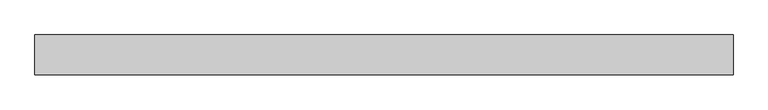
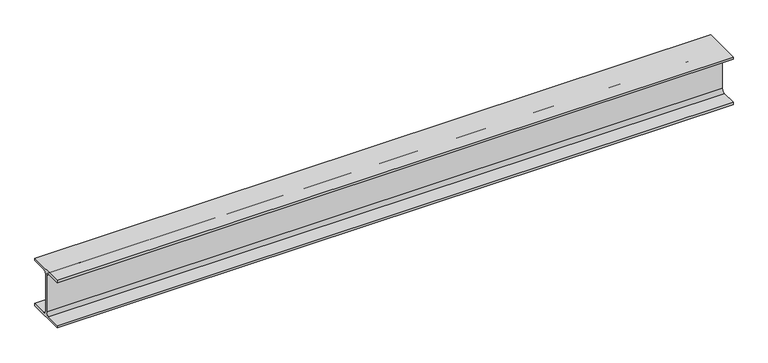
"""IFC4 building model written with IfcOpenShell, lengths in millimetres: beam geometry, 0912_Steel Framing_H-KSD3502 : H_SB_ASB_H-194x150x6x9."""

import ifcopenshell
import ifcopenshell.guid

model = None  # the IFC model being written
_history = None  # IfcOwnerHistory: only IFC2X3 demands one
_inside = {}  # id of a spatial element -> (the spatial element, [elements in it])
_under = {}  # id of a project, library or spatial element -> (it, [spatial elements below it])
_declared = {}  # id of a project -> (the project, [libraries it declares])
_typed = {}  # id of a type object -> (the type object, [elements of that type])
_made_of = {}  # id of a material, layer set ... -> (it, [elements and type objects made of it])


def new_model(schema):
    """Start an empty IFC model of exactly this schema.

    Asked for "IFC4X3", IfcOpenShell would pick the latest addendum, in which some entities
    have other attributes; the version numbers below select the first issue.
    IFC2X3 requires an IfcOwnerHistory on every rooted entity: one is made here for all.
    """
    global model, _history
    if schema == "IFC4X3":
        model = ifcopenshell.file(schema_version=(4, 3, 0, 0))
    else:
        model = ifcopenshell.file(schema=schema)
    _inside.clear()
    _under.clear()
    _declared.clear()
    _typed.clear()
    _made_of.clear()
    _history = None
    if model.schema == "IFC2X3":
        org = make("IfcOrganization", Name="unknown")
        user = make(
            "IfcPersonAndOrganization",
            ThePerson=make("IfcPerson", FamilyName="unknown"),
            TheOrganization=org,
        )
        app = make(
            "IfcApplication",
            ApplicationDeveloper=org,
            Version="unknown",
            ApplicationFullName="unknown",
            ApplicationIdentifier="unknown",
        )
        _history = make(
            "IfcOwnerHistory",
            OwningUser=user,
            OwningApplication=app,
            ChangeAction="ADDED",
            CreationDate=0,
        )
    return model


def make(cls, **values):
    """One entity of the class cls with the attributes given. An attribute that is None is left unset."""
    return model.create_entity(
        cls, **{name: value for name, value in values.items() if value is not None}
    )


def rooted(cls, **values):
    """An entity with a GlobalId (a new one), such as an element, a storey or a relation."""
    return make(cls, GlobalId=ifcopenshell.guid.new(), OwnerHistory=_history, **values)


def si_unit(unit_type, name, prefix=None):
    """IfcSIUnit, for example si_unit("LENGTHUNIT", "METRE", prefix="MILLI")."""
    return make("IfcSIUnit", UnitType=unit_type, Prefix=prefix, Name=name)


def assignment(units):
    """IfcUnitAssignment: the units of a project."""
    return None if units is None else make("IfcUnitAssignment", Units=units)


def point(xyz):
    """IfcCartesianPoint."""
    return None if xyz is None else make("IfcCartesianPoint", Coordinates=xyz)


def direction(xyz):
    """IfcDirection."""
    return None if xyz is None else make("IfcDirection", DirectionRatios=xyz)


def frame(location, z_axis=None, x_axis=None):
    """IfcAxis2Placement3D, a coordinate frame: its origin and axes. An axis left out is left unset."""
    return make(
        "IfcAxis2Placement3D",
        Location=point(location),
        Axis=direction(z_axis),
        RefDirection=direction(x_axis),
    )


def frame_2d(location, x_axis=None):
    """IfcAxis2Placement2D, a coordinate frame in the plane: its origin and x axis."""
    return make(
        "IfcAxis2Placement2D", Location=point(location), RefDirection=direction(x_axis)
    )


def origin():
    """The frame at (0, 0, 0) with its axes left unset."""
    return frame((0.0, 0.0, 0.0))


def place(relative_to, where):
    """IfcLocalPlacement: puts the frame where relative to a parent placement (None: the world)."""
    return make(
        "IfcLocalPlacement", PlacementRelTo=relative_to, RelativePlacement=where
    )


def context(
    kind, dimensions, precision=None, world=None, true_north=None, identifier=None
):
    """IfcGeometricRepresentationContext, for example the 3D "Model" context."""
    return make(
        "IfcGeometricRepresentationContext",
        ContextIdentifier=identifier,
        ContextType=kind,
        CoordinateSpaceDimension=dimensions,
        Precision=precision,
        WorldCoordinateSystem=world,
        TrueNorth=true_north,
    )


def project(units=None, contexts=None):
    """IfcProject with its units and contexts."""
    return rooted(
        "IfcProject",
        Name="project",
        RepresentationContexts=contexts,
        UnitsInContext=assignment(units),
    )


def spatial(cls, under=None, at=None, **own):
    """A site, building, storey or space (cls), placed at a placement, below another one or the project."""
    s = rooted(cls, ObjectPlacement=at, **own)
    if under is not None:
        _under.setdefault(under.id(), (under, []))[1].append(s)
    return s


def polyline(points):
    """IfcPolyline through the points."""
    return make("IfcPolyline", Points=[point(p) for p in points])


def circle_curve(where, radius):
    """IfcCircle in the frame where."""
    return make("IfcCircle", Position=where, Radius=radius)


def trimmed(basis, trim1, trim2, sense, master):
    """IfcTrimmedCurve: the piece of a basis curve between two trims."""
    return make(
        "IfcTrimmedCurve",
        BasisCurve=basis,
        Trim1=trim1,
        Trim2=trim2,
        SenseAgreement=sense,
        MasterRepresentation=master,
    )


def segment(curve, same_sense, transition):
    """IfcCompositeCurveSegment."""
    return make(
        "IfcCompositeCurveSegment",
        Transition=transition,
        SameSense=same_sense,
        ParentCurve=curve,
    )


def composite_curve(segments, self_intersect=None):
    """IfcCompositeCurve: segments joined end to end."""
    return make("IfcCompositeCurve", Segments=segments, SelfIntersect=self_intersect)


def outline(outer, holes=None, kind="AREA"):
    """IfcArbitraryClosedProfileDef: a profile drawn as a closed curve; with holes, ...WithVoids."""
    if holes is None:
        return make("IfcArbitraryClosedProfileDef", ProfileType=kind, OuterCurve=outer)
    return make(
        "IfcArbitraryProfileDefWithVoids",
        ProfileType=kind,
        OuterCurve=outer,
        InnerCurves=holes,
    )


def extrude(swept, where, along, depth):
    """IfcExtrudedAreaSolid: the profile swept, set in the frame where, extruded along a direction by depth."""
    return make(
        "IfcExtrudedAreaSolid",
        SweptArea=swept,
        Position=where,
        ExtrudedDirection=direction(along),
        Depth=depth,
    )


def shape(context_of_items, identifier, shape_type, items):
    """IfcShapeRepresentation: the items that make up one representation, for example the "Body"."""
    return make(
        "IfcShapeRepresentation",
        ContextOfItems=context_of_items,
        RepresentationIdentifier=identifier,
        RepresentationType=shape_type,
        Items=items,
    )


def source(mapping_origin, context_of_items, identifier, shape_type, items):
    """IfcRepresentationMap: a shape defined once, which mapped items show again and again."""
    return make(
        "IfcRepresentationMap",
        MappingOrigin=mapping_origin,
        MappedRepresentation=shape(context_of_items, identifier, shape_type, items),
    )


def transform(
    local_origin,
    x_axis=None,
    y_axis=None,
    z_axis=None,
    scale=None,
    scale2=None,
    scale3=None,
    uniform=True,
):
    """IfcCartesianTransformationOperator3D, or its non-uniform kind. x_axis, y_axis, z_axis: its Axis1, 2, 3."""
    if uniform:
        return make(
            "IfcCartesianTransformationOperator3D",
            Axis1=direction(x_axis),
            Axis2=direction(y_axis),
            LocalOrigin=point(local_origin),
            Scale=scale,
            Axis3=direction(z_axis),
        )
    return make(
        "IfcCartesianTransformationOperator3DnonUniform",
        Axis1=direction(x_axis),
        Axis2=direction(y_axis),
        LocalOrigin=point(local_origin),
        Scale=scale,
        Axis3=direction(z_axis),
        Scale2=scale2,
        Scale3=scale3,
    )


def mapped(mapping_source, mapping_target):
    """IfcMappedItem: shows the shape of a source again, moved by a transform."""
    return make(
        "IfcMappedItem", MappingSource=mapping_source, MappingTarget=mapping_target
    )


def made_of(thing, what):
    """Note that an element or type object is made of a material, layer set ...; save() writes the relation."""
    if what is not None:
        _made_of.setdefault(what.id(), (what, []))[1].append(thing)
    return thing


def element(
    cls,
    number,
    at=None,
    inside=None,
    cuts=None,
    type_object=None,
    material=None,
    context=None,
    identifier="Body",
    shape_type=None,
    held_by="IfcProductDefinitionShape",
    body=None,
    shapes=None,
    **own,
):
    """One element of the class cls, such as IfcWall. Its Tag is "e" and its number.

    at: its placement. inside: the storey or other place that contains it. cuts: it is an
    opening in that element (IfcRelVoidsElement). A single representation is given by context,
    identifier, shape_type and body (its items); several are given by shapes. held_by: the class
    of the entity that holds the representations. save() writes the other relations.
    """
    e = rooted(cls, Tag="e%d" % number, ObjectPlacement=at, **own)
    if body is not None:
        shapes = [shape(context, identifier, shape_type, body)]
    if shapes is not None:
        e.Representation = make(held_by, Representations=shapes)
    if inside is not None:
        _inside.setdefault(inside.id(), (inside, []))[1].append(e)
    if cuts is not None:
        rooted(
            "IfcRelVoidsElement", RelatingBuildingElement=cuts, RelatedOpeningElement=e
        )
    if type_object is not None:
        _typed.setdefault(type_object.id(), (type_object, []))[1].append(e)
    return made_of(e, material)


def aggregate(whole, parts):
    """IfcRelAggregates: a whole, such as a stair, and the parts it consists of."""
    return rooted("IfcRelAggregates", RelatingObject=whole, RelatedObjects=parts)


def save(model, path):
    """Write the relations noted so far, then the file.

    IfcRelAggregates (storeys below a building ...), IfcRelContainedInSpatialStructure (elements
    in a storey), IfcRelDefinesByType, IfcRelAssociatesMaterial and IfcRelDeclares: one each for
    every whole, place, type object, material and project.
    """
    for whole, parts in _under.values():
        aggregate(whole, parts)
    for where, things in _inside.values():
        rooted(
            "IfcRelContainedInSpatialStructure",
            RelatedElements=things,
            RelatingStructure=where,
        )
    for kind, things in _typed.values():
        rooted("IfcRelDefinesByType", RelatedObjects=things, RelatingType=kind)
    for what, things in _made_of.values():
        rooted("IfcRelAssociatesMaterial", RelatedObjects=things, RelatingMaterial=what)
    for by, libraries in _declared.values():
        rooted("IfcRelDeclares", RelatingContext=by, RelatedDefinitions=libraries)
    model.write(path)


def beam_8b6bb364(model_context):
    return source(origin(), model_context, "Body", "SweptSolid", [
        extrude(outline(composite_curve([segment(polyline([(75.0, -88.0), (75.0, -97.0), (-75.0, -97.0), (-75.0, -88.0), (-16.0, -88.0)]), True, "CONTINUOUS"), segment(trimmed(circle_curve(frame_2d((-16.0, -75.0)), 13.0), [point((-16.0, -88.0))], [point((-3.0, -75.0))], True, "CARTESIAN"), True, "CONTINUOUS"), segment(polyline([(-3.0, -75.0), (-3.0, 75.0)]), True, "CONTINUOUS"), segment(trimmed(circle_curve(frame_2d((-16.0, 75.0)), 13.0), [point((-3.0, 75.0))], [point((-16.0, 88.0))], True, "CARTESIAN"), True, "CONTINUOUS"), segment(polyline([(-16.0, 88.0), (-75.0, 88.0), (-75.0, 97.0), (75.0, 97.0), (75.0, 88.0), (16.0, 88.0)]), True, "CONTINUOUS"), segment(trimmed(circle_curve(frame_2d((16.0, 75.0)), 13.0), [point((16.0, 88.0))], [point((3.0, 75.0))], True, "CARTESIAN"), True, "CONTINUOUS"), segment(polyline([(3.0, 75.0), (3.0, -75.0)]), True, "CONTINUOUS"), segment(trimmed(circle_curve(frame_2d((16.0, -75.0)), 13.0), [point((3.0, -75.0))], [point((16.0, -88.0))], True, "CARTESIAN"), True, "CONTINUOUS"), segment(polyline([(16.0, -88.0), (75.0, -88.0)]), True, "CONTINUOUS")], self_intersect=False)), frame((-1068.0314701, 0.0, 0.0), z_axis=(1.0, 0.0, 0.0), x_axis=(0.0, 1.0, 0.0)), (0.0, 0.0, 1.0), 2617.0588612),
    ])


if __name__ == "__main__":
    model = new_model("IFC4")
    model_context = context("Model", 3, world=origin())
    ifc_project = project(units=[si_unit("LENGTHUNIT", "METRE", prefix="MILLI")], contexts=[model_context])
    site = spatial("IfcSite", under=ifc_project)
    building = spatial("IfcBuilding", under=site)
    placement = place(None, origin())
    beam_shape = beam_8b6bb364(model_context)
    element("IfcBeam", 1, ObjectType="0912_Steel Framing_H-KSD3502 : H_SB_ASB_H-194x150x6x9", at=placement, inside=building, context=model_context, shape_type="MappedRepresentation", body=[
        mapped(beam_shape, transform((0.0, 0.0, 0.0), x_axis=(1.0, 0.0, 0.0), y_axis=(0.0, 1.0, 0.0), z_axis=(0.0, 0.0, 1.0))),
    ])
    save(model, "model.ifc")

# Revit data of these elements
# Type "0912_Steel Framing_H-KSD3502 : H_SB_ASB_H-194x150x6x9"
#   H_WM Code_1 = "S01AA002-00001 | Main Steel Structure Fabrication Work | Shelter/Building | Medium Steel - Standard (90KG/M>Weight≥30KG/M) | Material: (   )"
#   H_WM Code_2 = "S03AA028-00001 | Main Steel Structure Erection Work | Shelter/Building | Medium Steel (90KG/M>Weight≥30KG/M) | Material: (   )"
#   H_WM Code_3 = "S01AA010-00001 | Main Steel Structure Fabrication Work | Shelter/Building | Steel Painting/Coating | for Non-Fireproofed Steel Surface, Surface Preparation, Primer, Second & Final Coat | Material: (   )"
#   H_Q'ty Cal Type Tag = "SB-Q2"
#   Width = 15.0 cm
#   Web Thickness = 0.6 cm
#   Web Fillet = 1.3 cm
#   Warping Constant = 43316.0 cm⁶
#   W = 0
#   Torsional Moment of Inertia = 8.622 cm⁴
#   Section Area = 39.01 cm²
#   Plastic Modulus weak axis = 104.0 cm³
#   Plastic Modulus strong axis = 309.0 cm³
#   Perimeter = 0.95 m²/m
#   Nominal Weight = 30.60 kgf/m
#   Moment of Inertia weak axis = 507.00 cm⁴
#   Moment of Inertia strong axis = 2690.00 cm⁴
#   Height = 19.4 cm
#   Flange Thickness = 0.9 cm
#   Elastic Modulus weak axis = 67.6 cm³
#   Elastic Modulus strong axis = 277.0 cm³
#   Centroid Vertical = 9.7 cm
#   Centroid Horizontal = 7.5 cm
#   Ix = 26900000
#   Length [instance default] = 1.5240 m
#   Zx = 309000
#   b = 0.1500 m
#   h = 0.1940 m
#   r = 0.0130 m
#   s = 0.0060 m
#   t = 0.0090 m
#   A = 0.003901 m²
#   Structural Material [instance default] = Steel, 45-345
#   Assembly Code = ""
# Element 1 (IfcBeam, "0912_Steel Framing_H-KSD3502 : H_SB_ASB_H-194x150x6x9")
#   Structural Material = none
# Materials
#   "Steel, 45-345": class "Metal", colour RGB 189 187 185, transparency 0, Description = "Steel 345 MPa", Cost = 0
